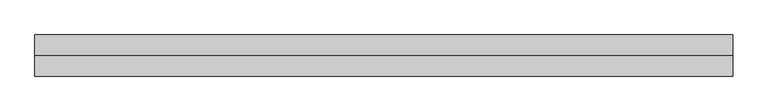
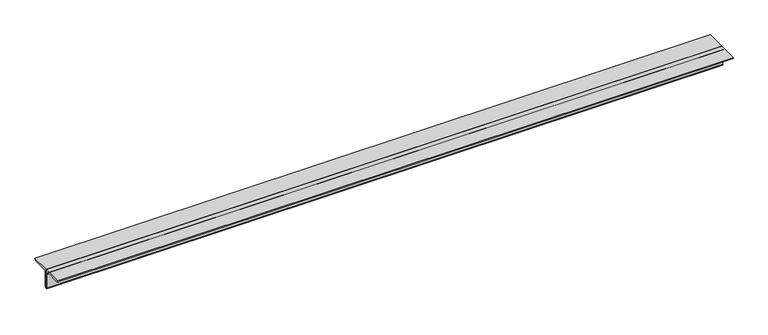
"""IFC4 building model written with IfcOpenShell, lengths in millimetres: member geometry, 0123_Steel Framing_2Ls-KSD3502 : H_SB_AR_S03_2Ls-130x130x12_HBR1."""

from ifc_helpers import new_model, si_unit, point, frame, frame_2d, origin, place, context, project, spatial, polyline, circle_curve, trimmed, segment, composite_curve, outline, extrude, source, transform, mapped, element, save


def member_ca2497e9(model_context):
    return source(origin(), model_context, "Body", "SweptSolid", [
        extrude(outline(composite_curve([segment(polyline([(0.0, 36.4), (130.0, 36.4)]), True, "CONTINUOUS"), segment(trimmed(circle_curve(frame_2d((118.0, 36.4)), 12.0), [point((130.0, 36.4))], [point((118.0, 24.4))], False, "CARTESIAN"), True, "CONTINUOUS"), segment(polyline([(118.0, 24.4), (24.0, 24.4)]), True, "CONTINUOUS"), segment(trimmed(circle_curve(frame_2d((24.0, 12.4)), 12.0), [point((24.0, 24.4))], [point((12.0, 12.4))], True, "CARTESIAN"), True, "CONTINUOUS"), segment(polyline([(12.0, 12.4), (12.0, -81.6)]), True, "CONTINUOUS"), segment(trimmed(circle_curve(frame_2d((0.0, -81.6)), 12.0), [point((12.0, -81.6))], [point((0.0, -93.6))], False, "CARTESIAN"), True, "CONTINUOUS"), segment(polyline([(0.0, -93.6), (0.0, 36.4)]), True, "CONTINUOUS")], self_intersect=False)), frame((-2209.5676318, 0.0, 0.0), z_axis=(1.0, 0.0, 0.0), x_axis=(0.0, 1.0, 0.0)), (0.0, 0.0, 1.0), 4412.2019305),
        extrude(outline(composite_curve([segment(polyline([(0.0, 36.4), (0.0, -93.6)]), True, "CONTINUOUS"), segment(trimmed(circle_curve(frame_2d((0.0, -81.6)), 12.0), [point((0.0, -93.6))], [point((-12.0, -81.6))], False, "CARTESIAN"), True, "CONTINUOUS"), segment(polyline([(-12.0, -81.6), (-12.0, 12.4)]), True, "CONTINUOUS"), segment(trimmed(circle_curve(frame_2d((-24.0, 12.4)), 12.0), [point((-12.0, 12.4))], [point((-24.0, 24.4))], True, "CARTESIAN"), True, "CONTINUOUS"), segment(polyline([(-24.0, 24.4), (-118.0, 24.4)]), True, "CONTINUOUS"), segment(trimmed(circle_curve(frame_2d((-118.0, 36.4)), 12.0), [point((-118.0, 24.4))], [point((-130.0, 36.4))], False, "CARTESIAN"), True, "CONTINUOUS"), segment(polyline([(-130.0, 36.4), (0.0, 36.4)]), True, "CONTINUOUS")], self_intersect=False)), frame((-2209.5676318, 0.0, 0.0), z_axis=(1.0, 0.0, 0.0), x_axis=(0.0, 1.0, 0.0)), (0.0, 0.0, 1.0), 4412.2019305),
    ])


if __name__ == "__main__":
    model = new_model("IFC4")
    model_context = context("Model", 3, world=origin())
    ifc_project = project(units=[si_unit("LENGTHUNIT", "METRE", prefix="MILLI")], contexts=[model_context])
    site = spatial("IfcSite", under=ifc_project)
    building = spatial("IfcBuilding", under=site)
    placement = place(None, origin())
    member_shape = member_ca2497e9(model_context)
    element("IfcMember", 1, ObjectType="0123_Steel Framing_2Ls-KSD3502 : H_SB_AR_S03_2Ls-130x130x12_HBR1", at=placement, inside=building, context=model_context, shape_type="MappedRepresentation", body=[
        mapped(member_shape, transform((0.0, 0.0, 0.0), x_axis=(1.0, 0.0, 0.0), y_axis=(0.0, 1.0, 0.0), z_axis=(0.0, 0.0, 1.0))),
    ])
    save(model, "model.ifc")

# Revit data of these elements
# Type "0123_Steel Framing_2Ls-KSD3502 : H_SB_AR_S03_2Ls-130x130x12_HBR1"
#   Type Mark = "HBR1"
#   Assembly Code = "B10"
#   Legs = "SLBB"
#   W = 8.97
#   Perimeter = 1.04 m²/m
#   Nominal Weight = 46.80 kgf/m
#   Length [instance default] = 1000 mm
#   Space = 0 mm
#   b = 130 mm
#   d = 130 mm
#   t = 12 mm
#   y = 36.4 mm
#   A = 0.005952 m²
#   Structural Material [instance default] = Steel ASTM A36
# Element 1 (IfcMember, "0123_Steel Framing_2Ls-KSD3502 : H_SB_AR_S03_2Ls-130x130x12_HBR1")
#   Materials on its faces: "Steel ASTM A36"
# Materials
#   "Steel ASTM A36": class "Metal", colour RGB 199 199 199, transparency 0, Description = "Structural steel, ASTM A36 Grade B, mill finish", Cost = 0
